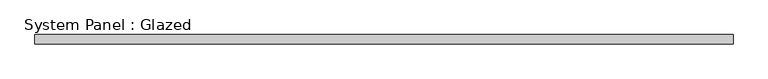
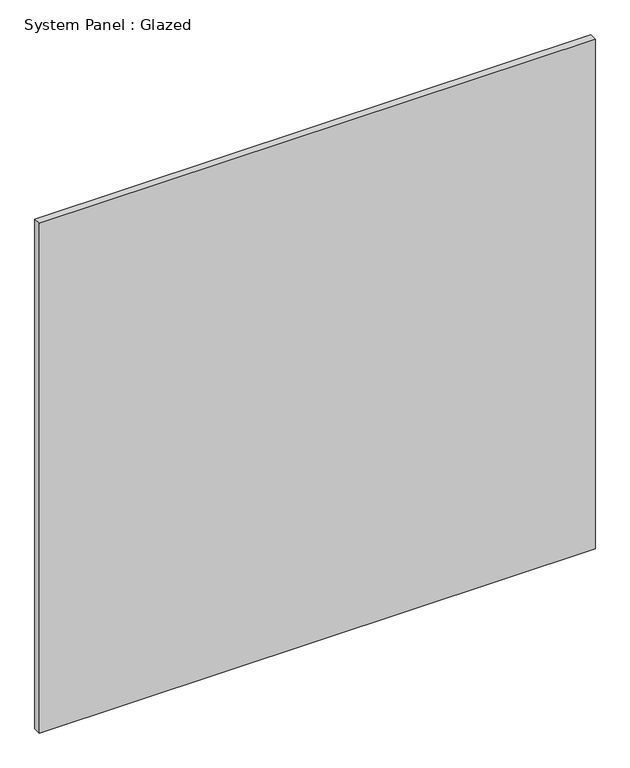
"""IFC4 building model written with IfcOpenShell, lengths in millimetres: plate geometry, System Panel : Glazed."""

from ifc_helpers import new_model, si_unit, origin, origin_with_axes, place, context, project, spatial, polyline, outline, extrude, source, transform, mapped, element, save


def system_panel_glazed_0c53a7ba(model_context):
    return source(origin(), model_context, "Body", "SweptSolid", [
        extrude(outline(polyline([(915.0000002, 24.5), (-915.0000002, 24.5), (-915.0000002, 49.5), (915.0000002, 49.5), (915.0000002, 24.5)])), origin_with_axes(), (0.0, 0.0, 1.0), 1772.3836314),
    ])


if __name__ == "__main__":
    model = new_model("IFC4")
    model_context = context("Model", 3, world=origin())
    ifc_project = project(units=[si_unit("LENGTHUNIT", "METRE", prefix="MILLI")], contexts=[model_context])
    site = spatial("IfcSite", under=ifc_project)
    building = spatial("IfcBuilding", under=site)
    placement = place(None, origin())
    system_panel_glazed_shape = system_panel_glazed_0c53a7ba(model_context)
    element("IfcPlate", 1, ObjectType="System Panel : Glazed", at=placement, inside=building, context=model_context, shape_type="MappedRepresentation", body=[
        mapped(system_panel_glazed_shape, transform((0.0, 0.0, 0.0), x_axis=(1.0, 0.0, 0.0), y_axis=(0.0, 1.0, 0.0), z_axis=(0.0, 0.0, 1.0))),
    ])
    save(model, "model.ifc")

# Revit data of these elements
# Element 1 (IfcPlate, "System Panel : Glazed")
#   Materials on its faces: "Glass"
# Materials
#   "Glass": class "Glass", colour RGB 218 227 224, transparency 0.85, Description = "Soda Lime Glass", Cost = 0
